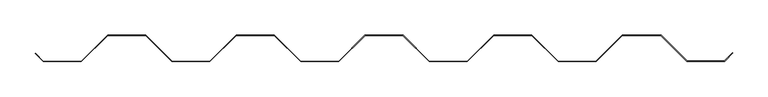
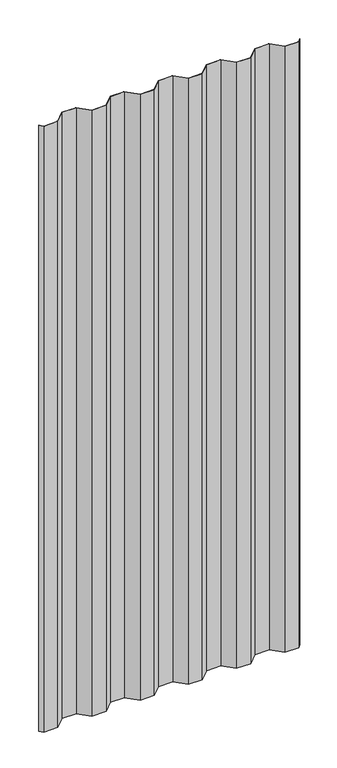
"""IFC4 building model written with IfcOpenShell, lengths in millimetres: proxy geometry, MBCI 7.2-V Panel2 : MBCI 7.2-V Panel-1."""

from ifc_helpers import new_model, si_unit, frame, origin, place, context, project, spatial, polyline, outline, extrude, source, transform, mapped, element, save


def generic_models_5825bab2(model_context):
    return source(origin(), model_context, "Body", "SweptSolid", [
        extrude(outline(polyline([(588241.1303729, -531639.2163841), (588187.0186638, -531639.2163841), (588175.6180296, -531627.81575), (588176.4180038, -531627.7738251), (588187.2652503, -531638.6210716), (588240.8837864, -531638.6210716), (588278.3741864, -531601.1306716), (588332.6548503, -531601.1306716), (588370.1452503, -531638.6210716), (588423.7637864, -531638.6210716), (588461.2541864, -531601.1306716), (588515.5348503, -531601.1306716), (588553.0252503, -531638.6210716), (588606.6437864, -531638.6210716), (588644.1341864, -531601.1306716), (588698.4148503, -531601.1306716), (588735.9052503, -531638.6210716), (588789.5237864, -531638.6210716), (588827.0141864, -531601.1306716), (588881.2948503, -531601.1306716), (588918.7852503, -531638.6210716), (588972.4037864, -531638.6210716), (589009.8941864, -531601.1306716), (589065.0384503, -531601.1306716), (589101.9192503, -531638.0114716), (589155.0073773, -531638.0114716), (589166.1378112, -531626.8810377), (589166.9246865, -531626.9360614), (589155.2539638, -531638.6067841), (589101.6726638, -531638.6067841), (589064.7918638, -531601.7259841), (589010.1407729, -531601.7259841), (588972.6503729, -531639.2163841), (588918.5386638, -531639.2163841), (588881.0482638, -531601.7259841), (588827.2607729, -531601.7259841), (588789.7703729, -531639.2163841), (588735.6586638, -531639.2163841), (588698.1682638, -531601.7259841), (588644.3807729, -531601.7259841), (588606.8903729, -531639.2163841), (588552.7786638, -531639.2163841), (588515.2882638, -531601.7259841), (588461.5007729, -531601.7259841), (588424.0103729, -531639.2163841), (588369.8986638, -531639.2163841), (588332.4082638, -531601.7259841), (588278.6207729, -531601.7259841), (588241.1303729, -531639.2163841)])), frame((0.0, 0.0, 6.35), z_axis=(0.0, 0.0, 1.0), x_axis=(1.0, 0.0, 0.0)), (0.0, 0.0, 1.0), 2432.05),
    ])


if __name__ == "__main__":
    model = new_model("IFC4")
    model_context = context("Model", 3, world=origin())
    ifc_project = project(units=[si_unit("LENGTHUNIT", "METRE", prefix="MILLI")], contexts=[model_context])
    site = spatial("IfcSite", under=ifc_project)
    building = spatial("IfcBuilding", under=site)
    placement = place(None, origin())
    generic_models_shape = generic_models_5825bab2(model_context)
    element("IfcBuildingElementProxy", 1, Name="MBCI 7.2-V Panel2 : MBCI 7.2-V Panel-1", ObjectType="MBCI 7.2-V Panel2 : MBCI 7.2-V Panel-1", at=placement, inside=building, context=model_context, shape_type="MappedRepresentation", body=[
        mapped(generic_models_shape, transform((0.0, 0.0, 0.0), x_axis=(1.0, 0.0, 0.0), y_axis=(0.0, 1.0, 0.0), z_axis=(0.0, 0.0, 1.0))),
    ])
    save(model, "model.ifc")

# Revit data of these elements
# Element 1 (IfcBuildingElementProxy, "MBCI 7.2-V Panel2 : MBCI 7.2-V Panel-1")
#   Materials on its faces: "MTL PANEL"
# Materials
#   "MTL PANEL": class "Generic", colour RGB 239 242 240, transparency 0, Cost = 0
